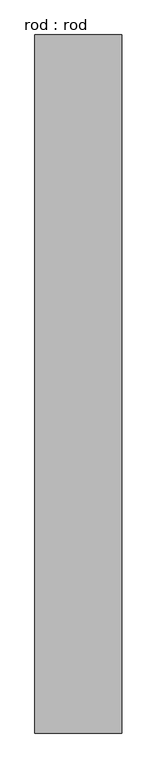
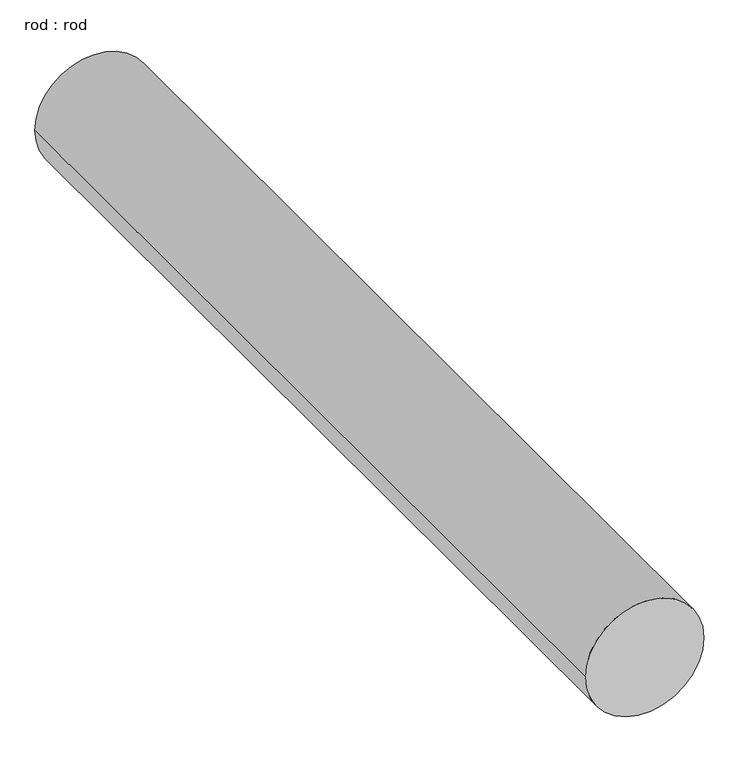
"""IFC4 building model written with IfcOpenShell, lengths in millimetres: proxy geometry, rod : rod."""

from ifc_helpers import new_model, si_unit, point, frame, frame_2d, origin, place, context, project, spatial, circle_curve, trimmed, segment, composite_curve, outline, extrude, source, transform, mapped, element, save


def rod_rod_bf28f6bd(model_context):
    return source(origin(), model_context, "Body", "SweptSolid", [
        extrude(outline(composite_curve([segment(trimmed(circle_curve(frame_2d((0.0108462, 0.0)), 200.0), [point((0.0108462, 200.0))], [point((0.0108462, -200.0))], False, "CARTESIAN"), True, "CONTINUOUS"), segment(trimmed(circle_curve(frame_2d((0.0108462, 0.0)), 200.0), [point((0.0108462, -200.0))], [point((0.0108462, 200.0))], False, "CARTESIAN"), True, "CONTINUOUS")], self_intersect=False)), frame((0.0, 2485.5857582, 0.0), z_axis=(0.0, 1.0, 0.0), x_axis=(0.0, 0.0, 1.0)), (0.0, 0.0, 1.0), 3214.2857143),
    ])


if __name__ == "__main__":
    model = new_model("IFC4")
    model_context = context("Model", 3, world=origin())
    ifc_project = project(units=[si_unit("LENGTHUNIT", "METRE", prefix="MILLI")], contexts=[model_context])
    site = spatial("IfcSite", under=ifc_project)
    building = spatial("IfcBuilding", under=site)
    placement = place(None, origin())
    rod_rod_shape = rod_rod_bf28f6bd(model_context)
    element("IfcBuildingElementProxy", 1, Name="rod : rod", ObjectType="rod : rod", at=placement, inside=building, context=model_context, shape_type="MappedRepresentation", body=[
        mapped(rod_rod_shape, transform((0.0, 0.0, 0.0), x_axis=(1.0, 0.0, 0.0), y_axis=(0.0, 1.0, 0.0), z_axis=(0.0, 0.0, 1.0))),
    ])
    save(model, "model.ifc")

# Revit data of these elements
# Type "rod : rod"
#   Default Elevation = 0
